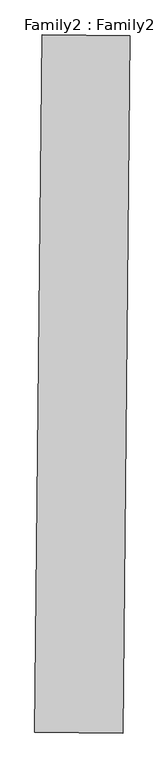
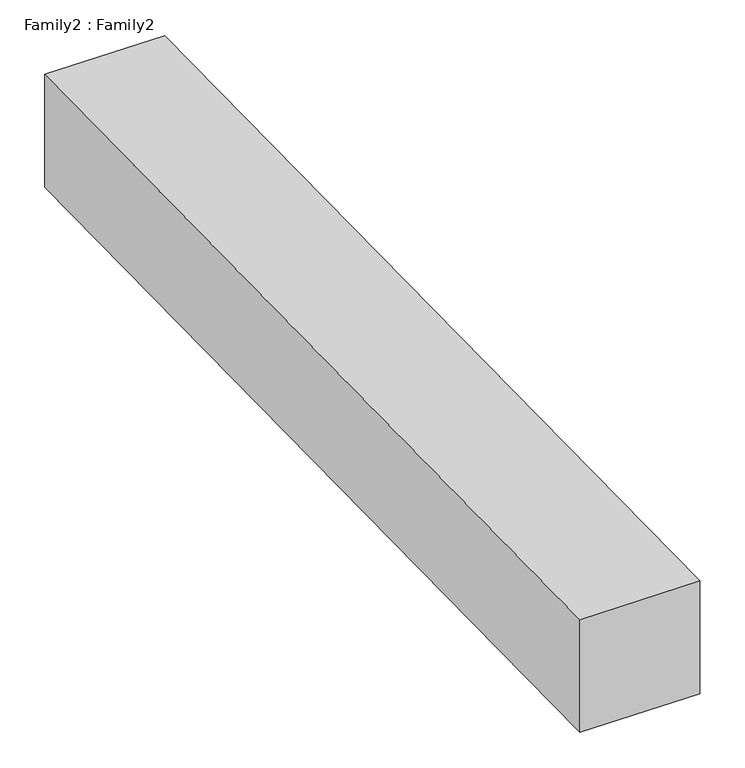
"""IFC4 building model written with IfcOpenShell, lengths in millimetres: proxy geometry, Family2 : Family2."""

from ifc_helpers import new_model, si_unit, origin, place, context, project, spatial, faceted_brep, source, transform, mapped, element, save


def family2_family2_10f01563(model_context):
    return source(origin(), model_context, "Body", "Brep", [
        faceted_brep([(-3951.6654125, -6865.3050411, 1.0945136), (-3951.6654125, -6865.3050411, 201.0945136), (-3935.177382, -5282.2950815, 202.060409), (-3935.177382, -5282.2950815, 2.060409), (-3751.6742225, -6867.1822537, 201.0945136), (-3735.186192, -5284.1722942, 202.060409), (-3751.6742225, -6867.1822537, 1.0945136), (-3735.186192, -5284.1722942, 2.060409)], [[[0, 1, 2, 3]], [[1, 4, 5, 2]], [[4, 6, 7, 5]], [[6, 0, 3, 7]], [[3, 2, 5, 7]], [[0, 6, 4, 1]]]),
    ])


if __name__ == "__main__":
    model = new_model("IFC4")
    model_context = context("Model", 3, world=origin())
    ifc_project = project(units=[si_unit("LENGTHUNIT", "METRE", prefix="MILLI")], contexts=[model_context])
    site = spatial("IfcSite", under=ifc_project)
    building = spatial("IfcBuilding", under=site)
    placement = place(None, origin())
    family2_family2_shape = family2_family2_10f01563(model_context)
    element("IfcBuildingElementProxy", 1, Name="Family2 : Family2", ObjectType="Family2 : Family2", at=placement, inside=building, context=model_context, shape_type="MappedRepresentation", body=[
        mapped(family2_family2_shape, transform((0.0, 0.0, 0.0), x_axis=(1.0, 0.0, 0.0), y_axis=(0.0, 1.0, 0.0), z_axis=(0.0, 0.0, 1.0))),
    ])
    save(model, "model.ifc")

# Revit data of these elements
# Type "Family2 : Family2"
#   Default Elevation = 0
